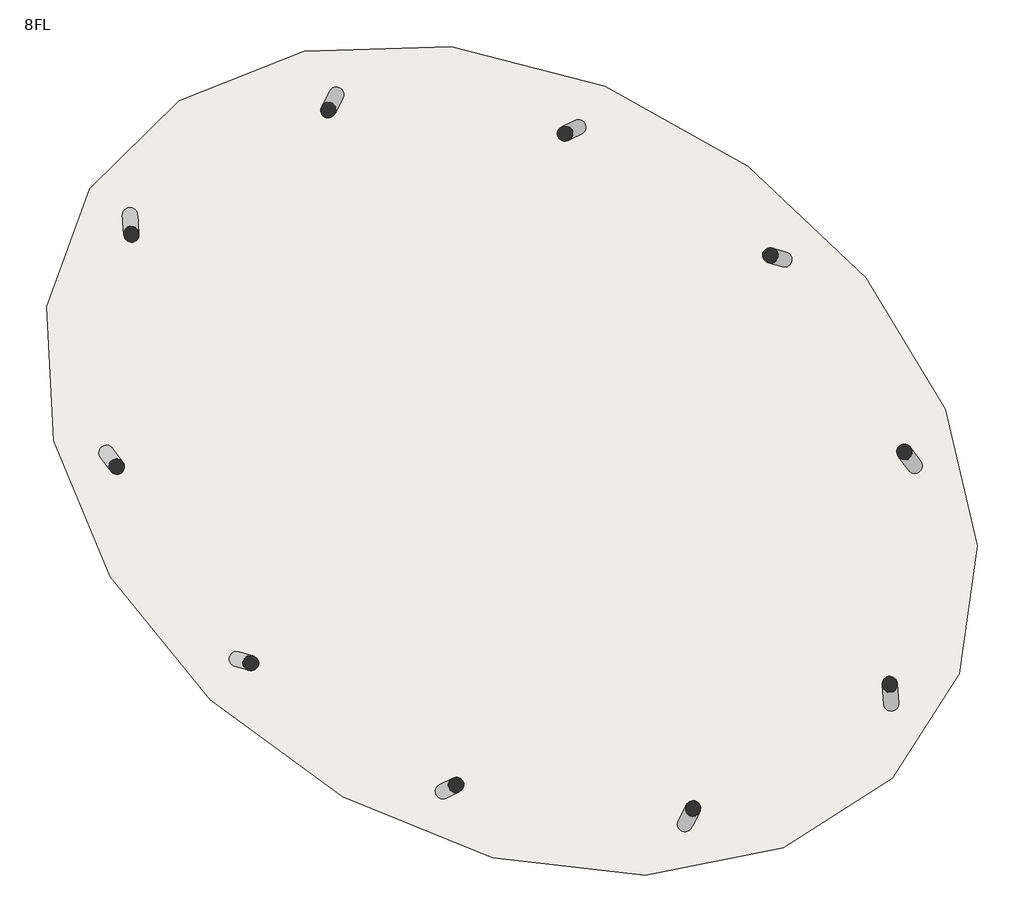
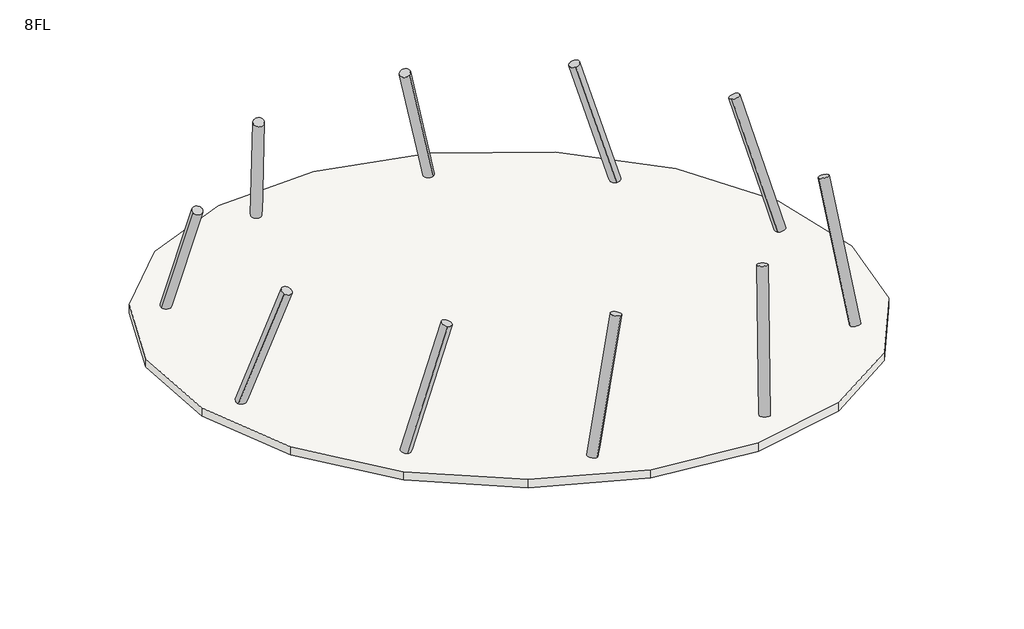
# One storey: 10 columns, 1 slab.
"""IFC4 building model written with IfcOpenShell, lengths in millimetres."""

from ifc_helpers import new_model, si_unit, point, frame, frame_2d, origin, place, context, project, spatial, polyline, circle_curve, trimmed, segment, composite_curve, outline, extrude, element, save

model = new_model("IFC4")

# Units and contexts
model_context = context("Model", 3, world=origin())
ifc_project = project(units=[si_unit("LENGTHUNIT", "METRE", prefix="MILLI")], contexts=[model_context])

# Site, building, storey
site = spatial("IfcSite", under=ifc_project)
building = spatial("IfcBuilding", under=site)
storey = spatial("IfcBuildingStorey", under=building, Name="8FL", Elevation=31500.0)

# Columns
placement = place(None, origin())
element("IfcColumn", 1, ObjectType="コンクリート-円形-柱 : 750", at=placement, inside=storey, context=model_context, shape_type="SweptSolid", body=[
    extrude(outline(composite_curve([segment(trimmed(circle_curve(frame_2d((0.0, -175.0000001)), 175.0), [point((0.0, -350.0))], [point((0.0, 0.0))], False, "CARTESIAN"), True, "CONTINUOUS"), segment(trimmed(circle_curve(frame_2d((0.0, -175.0000001)), 175.0), [point((0.0, 0.0))], [point((0.0, -350.0))], False, "CARTESIAN"), True, "CONTINUOUS")], self_intersect=False)), frame((-8623.1276881, 5666.7704224, 31500.0), z_axis=(0.02594195771459022, -0.35203237832536155, 0.9356282485263707), x_axis=(0.0687618312079851, -0.933098081666364, -0.35298694106082174)), (0.0, 0.0, 1.0), 4809.6025393),
])
element("IfcColumn", 2, ObjectType="コンクリート-円形-柱 : 750", at=placement, inside=storey, context=model_context, shape_type="SweptSolid", body=[
    extrude(outline(composite_curve([segment(trimmed(circle_curve(frame_2d((0.0, -175.0)), 175.0), [point((0.0, -350.0))], [point((0.0, 0.0))], False, "CARTESIAN"), True, "CONTINUOUS"), segment(trimmed(circle_curve(frame_2d((0.0, -175.0)), 175.0), [point((0.0, 0.0))], [point((0.0, -350.0))], False, "CARTESIAN"), True, "CONTINUOUS")], self_intersect=False)), frame((-9205.2482787, 261.1344657, 31500.0), z_axis=(0.18976265672131148, -0.2569549801170849, 0.9476097679462251), x_axis=(0.5629426428517169, -0.7622728206923179, -0.31943031742917233)), (0.0, 0.0, 1.0), 4748.7902217),
])
element("IfcColumn", 3, ObjectType="コンクリート-円形-柱 : 750", at=placement, inside=storey, context=model_context, shape_type="SweptSolid", body=[
    extrude(outline(composite_curve([segment(trimmed(circle_curve(frame_2d((0.0, -175.0)), 175.0), [point((0.0, -349.9999999))], [point((0.0, 0.0))], False, "CARTESIAN"), True, "CONTINUOUS"), segment(trimmed(circle_curve(frame_2d((0.0, -175.0)), 175.0), [point((0.0, 0.0))], [point((0.0, -349.9999999))], False, "CARTESIAN"), True, "CONTINUOUS")], self_intersect=False)), frame((-6284.7604037, -4447.7761387, 31500.0), z_axis=(0.2625861776754821, -0.07562058928306084, 0.9619407600108558), x_axis=(0.924372864586551, -0.26620449467714974, -0.2732580725792693)), (0.0, 0.0, 1.0), 4678.0427518),
])
element("IfcColumn", 4, ObjectType="コンクリート-円形-柱 : 750", at=placement, inside=storey, context=model_context, shape_type="SweptSolid", body=[
    extrude(outline(composite_curve([segment(trimmed(circle_curve(frame_2d((0.0, -174.9999999)), 175.0), [point((-1e-07, -350.0))], [point((0.0, 0.0))], False, "CARTESIAN"), True, "CONTINUOUS"), segment(trimmed(circle_curve(frame_2d((0.0, -174.9999999)), 175.0), [point((0.0, 0.0))], [point((-1e-07, -350.0))], False, "CARTESIAN"), True, "CONTINUOUS")], self_intersect=False)), frame((-1644.9139825, -7521.25735, 31500.0), z_axis=(0.24678218418133743, 0.12093320483037363, 0.9614955608530615), x_axis=(0.863399954513249, 0.42310073515259117, -0.27482046222917367)), (0.0, 0.0, 1.0), 4680.2088236),
])
element("IfcColumn", 5, ObjectType="コンクリート-円形-柱 : 750", at=placement, inside=storey, context=model_context, shape_type="SweptSolid", body=[
    extrude(outline(composite_curve([segment(trimmed(circle_curve(frame_2d((0.0, -175.0)), 175.0), [point((0.0, -350.0))], [point((0.0, 0.0))], False, "CARTESIAN"), True, "CONTINUOUS"), segment(trimmed(circle_curve(frame_2d((0.0, -175.0)), 175.0), [point((0.0, 0.0))], [point((0.0, -350.0))], False, "CARTESIAN"), True, "CONTINUOUS")], self_intersect=False)), frame((3869.9655392, -8355.8329726, 31500.0), z_axis=(0.14758177857760413, 0.285703612271388, 0.9468859828759487), x_axis=(0.4345658490594893, 0.84127616595156, -0.321569487720848)), (0.0, 0.0, 1.0), 4752.4201303),
])
element("IfcColumn", 6, ObjectType="コンクリート-円形-柱 : 750", at=placement, inside=storey, context=model_context, shape_type="SweptSolid", body=[
    extrude(outline(composite_curve([segment(trimmed(circle_curve(frame_2d((0.0, -175.0)), 175.0), [point((1e-07, -350.0))], [point((0.0, 0.0))], False, "CARTESIAN"), True, "CONTINUOUS"), segment(trimmed(circle_curve(frame_2d((0.0, -175.0)), 175.0), [point((0.0, 0.0))], [point((1e-07, -350.0))], False, "CARTESIAN"), True, "CONTINUOUS")], self_intersect=False)), frame((8623.1277206, -5666.770404, 31500.0), z_axis=(-0.02594195863279733, 0.35203237924746134, 0.9356282481539694), x_axis=(-0.06876183342213427, 0.9330980811297881, -0.35298694204790954)), (0.0, 0.0, 1.0), 4809.6025393),
])
element("IfcColumn", 7, ObjectType="コンクリート-円形-柱 : 750", at=placement, inside=storey, context=model_context, shape_type="SweptSolid", body=[
    extrude(outline(composite_curve([segment(trimmed(circle_curve(frame_2d((0.0, -175.0000001)), 175.0), [point((0.0, -350.0))], [point((0.0, 0.0))], False, "CARTESIAN"), True, "CONTINUOUS"), segment(trimmed(circle_curve(frame_2d((0.0, -175.0000001)), 175.0), [point((0.0, 0.0))], [point((0.0, -350.0))], False, "CARTESIAN"), True, "CONTINUOUS")], self_intersect=False)), frame((9205.2482632, -261.1344467, 31500.0), z_axis=(-0.1897626605637729, 0.2569549810909145, 0.9476097669126919), x_axis=(-0.5629426482332456, 0.762272815433206, -0.3194303204952121)), (0.0, 0.0, 1.0), 4748.7902217),
])
element("IfcColumn", 8, ObjectType="コンクリート-円形-柱 : 750", at=placement, inside=storey, context=model_context, shape_type="SweptSolid", body=[
    extrude(outline(composite_curve([segment(trimmed(circle_curve(frame_2d((1e-07, -175.0)), 175.0), [point((0.0, -350.0))], [point((0.0, 0.0))], False, "CARTESIAN"), True, "CONTINUOUS"), segment(trimmed(circle_curve(frame_2d((1e-07, -175.0)), 175.0), [point((0.0, 0.0))], [point((0.0, -350.0))], False, "CARTESIAN"), True, "CONTINUOUS")], self_intersect=False)), frame((6284.7603761, 4447.776144, 31500.0), z_axis=(-0.26258618038263226, 0.075620589927825, 0.9619407592211839), x_axis=(-0.9243728639539592, 0.2662044940202606, -0.2732580753591238)), (0.0, 0.0, 1.0), 4678.0427518),
])
element("IfcColumn", 9, ObjectType="コンクリート-円形-柱 : 750", at=placement, inside=storey, context=model_context, shape_type="SweptSolid", body=[
    extrude(outline(composite_curve([segment(trimmed(circle_curve(frame_2d((1e-07, -175.0)), 175.0), [point((0.0, -350.0))], [point((0.0, 0.0))], False, "CARTESIAN"), True, "CONTINUOUS"), segment(trimmed(circle_curve(frame_2d((1e-07, -175.0)), 175.0), [point((0.0, 0.0))], [point((0.0, -350.0))], False, "CARTESIAN"), True, "CONTINUOUS")], self_intersect=False)), frame((1644.9140179, 7521.2573366, 31500.0), z_axis=(-0.24678219066542895, -0.12093320217729721, 0.9614955595225164), x_axis=(-0.8633999613790703, -0.42310071811820066, -0.274820466884261)), (0.0, 0.0, 1.0), 4680.2088236),
])
element("IfcColumn", 10, ObjectType="コンクリート-円形-柱 : 750", at=placement, inside=storey, context=model_context, shape_type="SweptSolid", body=[
    extrude(outline(composite_curve([segment(trimmed(circle_curve(frame_2d((0.0, -175.0)), 175.0), [point((0.0, -350.0))], [point((0.0, 0.0))], False, "CARTESIAN"), True, "CONTINUOUS"), segment(trimmed(circle_curve(frame_2d((0.0, -175.0)), 175.0), [point((0.0, 0.0))], [point((0.0, -350.0))], False, "CARTESIAN"), True, "CONTINUOUS")], self_intersect=False)), frame((-3869.9654679, 8355.8329895, 31500.0), z_axis=(-0.14758179079842773, -0.2857036109569364, 0.9468859813678187), x_axis=(-0.43456587835123517, -0.8412761491232924, -0.32156949216165287)), (0.0, 0.0, 1.0), 4752.4201303),
])

# Slab
element("IfcSlab", 11, ObjectType="一般 300 mm", at=placement, inside=storey, context=model_context, shape_type="SweptSolid", body=[
    extrude(outline(polyline([(-10558.9582223, 425.5161627), (-10726.1340166, 3526.7783801), (-9725.0904349, 6249.936122), (-7663.867557, 8291.7580013), (-4773.4128834, 9428.0004343), (-1371.4743124, 9540.5478276), (2175.0513437, 8622.2262218), (5485.7220506, 6774.145923), (8205.0984558, 4195.2551036), (10040.0490525, 1161.5569267), (10790.0523211, -2002.6148926), (10368.0487415, -4955.9058443), (8815.0936078, -7372.3511598), (6303.992314, -8983.0605413), (3114.1977635, -9615.2780409), (-407.6171905, -9206.3920578), (-3883.1285747, -7804.0702073), (-6939.5038642, -5560.2985152), (-9248.1185765, -2715.7498843), (-10558.9582223, 425.5161627)])), frame((0.0, 0.0, 31200.0), z_axis=(0.0, 0.0, 1.0), x_axis=(1.0, 0.0, 0.0)), (0.0, 0.0, 1.0), 300.0),
])

save(model, "model.ifc")

# Revit data of these elements
# Type "コンクリート-円形-柱 : 750"
#   Keynote = "03310.Q1"
#   R = 350 mm
#   Structural Material [instance default] = コンクリート - 現場打ち
# Type "一般 300 mm"
#   Function = 0
#   Layers, outside or top first: 300 mm no material (function 1)
# Elements 1, 2, 3, 4, 5, 6, 7, 8, 9, 10 (IfcColumn, "コンクリート-円形-柱 : 750")
#   Structural Material = コンクリート - 現場打ち
#   Phase Created = 新しい建設
#   Materials on its faces: "コンクリート - 現場打ち"
# Element 11 (IfcSlab, "一般 300 mm")
#   Height Offset From Level = 0 mm
#   Phase Created = 新しい建設
# Materials
#   "コンクリート - 現場打ち": class "コンクリート", colour RGB 192 192 192, transparency 0
